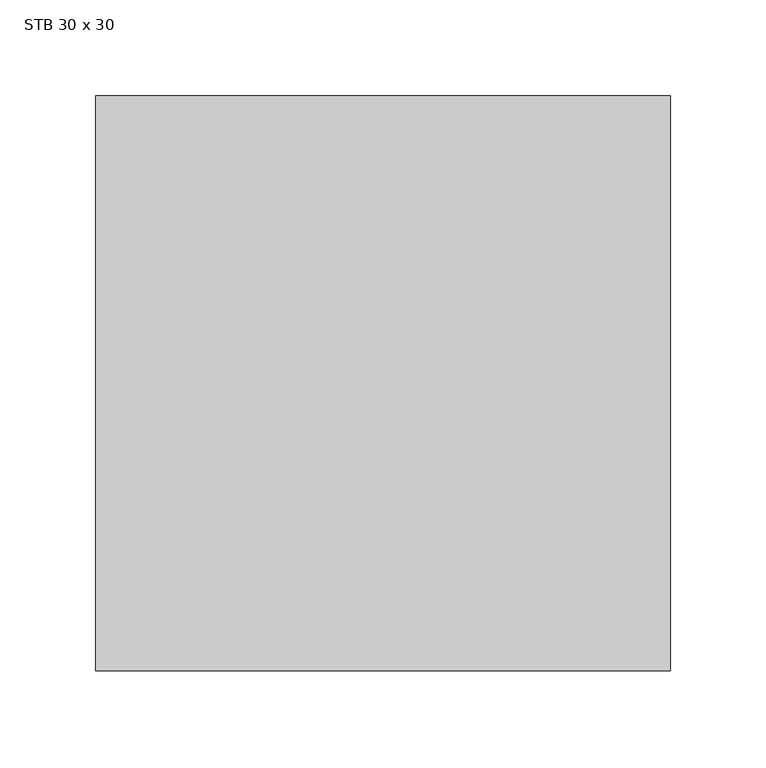
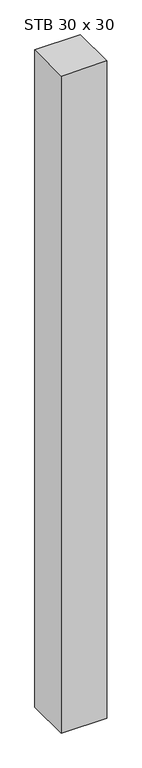
"""IFC4 building model written with IfcOpenShell, lengths in millimetres: column geometry, STB Stütze - rechteckig : STB 30 x 30."""

import ifcopenshell
import ifcopenshell.guid

model = None  # the IFC model being written
_history = None  # IfcOwnerHistory: only IFC2X3 demands one
_inside = {}  # id of a spatial element -> (the spatial element, [elements in it])
_under = {}  # id of a project, library or spatial element -> (it, [spatial elements below it])
_declared = {}  # id of a project -> (the project, [libraries it declares])
_typed = {}  # id of a type object -> (the type object, [elements of that type])
_made_of = {}  # id of a material, layer set ... -> (it, [elements and type objects made of it])


def new_model(schema):
    """Start an empty IFC model of exactly this schema.

    Asked for "IFC4X3", IfcOpenShell would pick the latest addendum, in which some entities
    have other attributes; the version numbers below select the first issue.
    IFC2X3 requires an IfcOwnerHistory on every rooted entity: one is made here for all.
    """
    global model, _history
    if schema == "IFC4X3":
        model = ifcopenshell.file(schema_version=(4, 3, 0, 0))
    else:
        model = ifcopenshell.file(schema=schema)
    _inside.clear()
    _under.clear()
    _declared.clear()
    _typed.clear()
    _made_of.clear()
    _history = None
    if model.schema == "IFC2X3":
        org = make("IfcOrganization", Name="unknown")
        user = make(
            "IfcPersonAndOrganization",
            ThePerson=make("IfcPerson", FamilyName="unknown"),
            TheOrganization=org,
        )
        app = make(
            "IfcApplication",
            ApplicationDeveloper=org,
            Version="unknown",
            ApplicationFullName="unknown",
            ApplicationIdentifier="unknown",
        )
        _history = make(
            "IfcOwnerHistory",
            OwningUser=user,
            OwningApplication=app,
            ChangeAction="ADDED",
            CreationDate=0,
        )
    return model


def make(cls, **values):
    """One entity of the class cls with the attributes given. An attribute that is None is left unset."""
    return model.create_entity(
        cls, **{name: value for name, value in values.items() if value is not None}
    )


def rooted(cls, **values):
    """An entity with a GlobalId (a new one), such as an element, a storey or a relation."""
    return make(cls, GlobalId=ifcopenshell.guid.new(), OwnerHistory=_history, **values)


def si_unit(unit_type, name, prefix=None):
    """IfcSIUnit, for example si_unit("LENGTHUNIT", "METRE", prefix="MILLI")."""
    return make("IfcSIUnit", UnitType=unit_type, Prefix=prefix, Name=name)


def assignment(units):
    """IfcUnitAssignment: the units of a project."""
    return None if units is None else make("IfcUnitAssignment", Units=units)


def point(xyz):
    """IfcCartesianPoint."""
    return None if xyz is None else make("IfcCartesianPoint", Coordinates=xyz)


def direction(xyz):
    """IfcDirection."""
    return None if xyz is None else make("IfcDirection", DirectionRatios=xyz)


def frame(location, z_axis=None, x_axis=None):
    """IfcAxis2Placement3D, a coordinate frame: its origin and axes. An axis left out is left unset."""
    return make(
        "IfcAxis2Placement3D",
        Location=point(location),
        Axis=direction(z_axis),
        RefDirection=direction(x_axis),
    )


def origin():
    """The frame at (0, 0, 0) with its axes left unset."""
    return frame((0.0, 0.0, 0.0))


def place(relative_to, where):
    """IfcLocalPlacement: puts the frame where relative to a parent placement (None: the world)."""
    return make(
        "IfcLocalPlacement", PlacementRelTo=relative_to, RelativePlacement=where
    )


def context(
    kind, dimensions, precision=None, world=None, true_north=None, identifier=None
):
    """IfcGeometricRepresentationContext, for example the 3D "Model" context."""
    return make(
        "IfcGeometricRepresentationContext",
        ContextIdentifier=identifier,
        ContextType=kind,
        CoordinateSpaceDimension=dimensions,
        Precision=precision,
        WorldCoordinateSystem=world,
        TrueNorth=true_north,
    )


def project(units=None, contexts=None):
    """IfcProject with its units and contexts."""
    return rooted(
        "IfcProject",
        Name="project",
        RepresentationContexts=contexts,
        UnitsInContext=assignment(units),
    )


def spatial(cls, under=None, at=None, **own):
    """A site, building, storey or space (cls), placed at a placement, below another one or the project."""
    s = rooted(cls, ObjectPlacement=at, **own)
    if under is not None:
        _under.setdefault(under.id(), (under, []))[1].append(s)
    return s


def polyline(points):
    """IfcPolyline through the points."""
    return make("IfcPolyline", Points=[point(p) for p in points])


def outline(outer, holes=None, kind="AREA"):
    """IfcArbitraryClosedProfileDef: a profile drawn as a closed curve; with holes, ...WithVoids."""
    if holes is None:
        return make("IfcArbitraryClosedProfileDef", ProfileType=kind, OuterCurve=outer)
    return make(
        "IfcArbitraryProfileDefWithVoids",
        ProfileType=kind,
        OuterCurve=outer,
        InnerCurves=holes,
    )


def extrude(swept, where, along, depth):
    """IfcExtrudedAreaSolid: the profile swept, set in the frame where, extruded along a direction by depth."""
    return make(
        "IfcExtrudedAreaSolid",
        SweptArea=swept,
        Position=where,
        ExtrudedDirection=direction(along),
        Depth=depth,
    )


def shape(context_of_items, identifier, shape_type, items):
    """IfcShapeRepresentation: the items that make up one representation, for example the "Body"."""
    return make(
        "IfcShapeRepresentation",
        ContextOfItems=context_of_items,
        RepresentationIdentifier=identifier,
        RepresentationType=shape_type,
        Items=items,
    )


def source(mapping_origin, context_of_items, identifier, shape_type, items):
    """IfcRepresentationMap: a shape defined once, which mapped items show again and again."""
    return make(
        "IfcRepresentationMap",
        MappingOrigin=mapping_origin,
        MappedRepresentation=shape(context_of_items, identifier, shape_type, items),
    )


def transform(
    local_origin,
    x_axis=None,
    y_axis=None,
    z_axis=None,
    scale=None,
    scale2=None,
    scale3=None,
    uniform=True,
):
    """IfcCartesianTransformationOperator3D, or its non-uniform kind. x_axis, y_axis, z_axis: its Axis1, 2, 3."""
    if uniform:
        return make(
            "IfcCartesianTransformationOperator3D",
            Axis1=direction(x_axis),
            Axis2=direction(y_axis),
            LocalOrigin=point(local_origin),
            Scale=scale,
            Axis3=direction(z_axis),
        )
    return make(
        "IfcCartesianTransformationOperator3DnonUniform",
        Axis1=direction(x_axis),
        Axis2=direction(y_axis),
        LocalOrigin=point(local_origin),
        Scale=scale,
        Axis3=direction(z_axis),
        Scale2=scale2,
        Scale3=scale3,
    )


def mapped(mapping_source, mapping_target):
    """IfcMappedItem: shows the shape of a source again, moved by a transform."""
    return make(
        "IfcMappedItem", MappingSource=mapping_source, MappingTarget=mapping_target
    )


def made_of(thing, what):
    """Note that an element or type object is made of a material, layer set ...; save() writes the relation."""
    if what is not None:
        _made_of.setdefault(what.id(), (what, []))[1].append(thing)
    return thing


def element(
    cls,
    number,
    at=None,
    inside=None,
    cuts=None,
    type_object=None,
    material=None,
    context=None,
    identifier="Body",
    shape_type=None,
    held_by="IfcProductDefinitionShape",
    body=None,
    shapes=None,
    **own,
):
    """One element of the class cls, such as IfcWall. Its Tag is "e" and its number.

    at: its placement. inside: the storey or other place that contains it. cuts: it is an
    opening in that element (IfcRelVoidsElement). A single representation is given by context,
    identifier, shape_type and body (its items); several are given by shapes. held_by: the class
    of the entity that holds the representations. save() writes the other relations.
    """
    e = rooted(cls, Tag="e%d" % number, ObjectPlacement=at, **own)
    if body is not None:
        shapes = [shape(context, identifier, shape_type, body)]
    if shapes is not None:
        e.Representation = make(held_by, Representations=shapes)
    if inside is not None:
        _inside.setdefault(inside.id(), (inside, []))[1].append(e)
    if cuts is not None:
        rooted(
            "IfcRelVoidsElement", RelatingBuildingElement=cuts, RelatedOpeningElement=e
        )
    if type_object is not None:
        _typed.setdefault(type_object.id(), (type_object, []))[1].append(e)
    return made_of(e, material)


def aggregate(whole, parts):
    """IfcRelAggregates: a whole, such as a stair, and the parts it consists of."""
    return rooted("IfcRelAggregates", RelatingObject=whole, RelatedObjects=parts)


def save(model, path):
    """Write the relations noted so far, then the file.

    IfcRelAggregates (storeys below a building ...), IfcRelContainedInSpatialStructure (elements
    in a storey), IfcRelDefinesByType, IfcRelAssociatesMaterial and IfcRelDeclares: one each for
    every whole, place, type object, material and project.
    """
    for whole, parts in _under.values():
        aggregate(whole, parts)
    for where, things in _inside.values():
        rooted(
            "IfcRelContainedInSpatialStructure",
            RelatedElements=things,
            RelatingStructure=where,
        )
    for kind, things in _typed.values():
        rooted("IfcRelDefinesByType", RelatedObjects=things, RelatingType=kind)
    for what, things in _made_of.values():
        rooted("IfcRelAssociatesMaterial", RelatedObjects=things, RelatingMaterial=what)
    for by, libraries in _declared.values():
        rooted("IfcRelDeclares", RelatingContext=by, RelatedDefinitions=libraries)
    model.write(path)


def stb_30_x_30_23a68b31(model_context):
    return source(origin(), model_context, "Body", "SweptSolid", [
        extrude(outline(polyline([(150.0, 150.0), (150.0, -150.0), (-150.0, -150.0), (-150.0, 150.0), (150.0, 150.0)])), frame((0.0, 0.0, -1584.8398838), z_axis=(0.0, 0.0, 1.0), x_axis=(1.0, 0.0, 0.0)), (0.0, 0.0, 1.0), 4584.8398838),
    ])


if __name__ == "__main__":
    model = new_model("IFC4")
    model_context = context("Model", 3, world=origin())
    ifc_project = project(units=[si_unit("LENGTHUNIT", "METRE", prefix="MILLI")], contexts=[model_context])
    site = spatial("IfcSite", under=ifc_project)
    building = spatial("IfcBuilding", under=site)
    placement = place(None, origin())
    stb_30_x_30_shape = stb_30_x_30_23a68b31(model_context)
    element("IfcColumn", 1, ObjectType="STB Stütze - rechteckig : STB 30 x 30", at=placement, inside=building, context=model_context, shape_type="MappedRepresentation", body=[
        mapped(stb_30_x_30_shape, transform((0.0, 0.0, 0.0), x_axis=(1.0, 0.0, 0.0), y_axis=(0.0, 1.0, 0.0), z_axis=(0.0, 0.0, 1.0))),
    ])
    save(model, "model.ifc")

# Revit data of these elements
# Type "STB Stütze - rechteckig : STB 30 x 30"
#   Breite = 0.300 m
#   Tiefe = 0.300 m
#   Structural Material [instance default] = Stahlbeton - Ortbeton
# Element 1 (IfcColumn, "STB Stütze - rechteckig : STB 30 x 30")
#   Materials on its faces: "Stahlbeton - Ortbeton"
# Materials
#   "Stahlbeton - Ortbeton": class "Beton", colour RGB 247 247 247, transparency 0, Cost = 0
